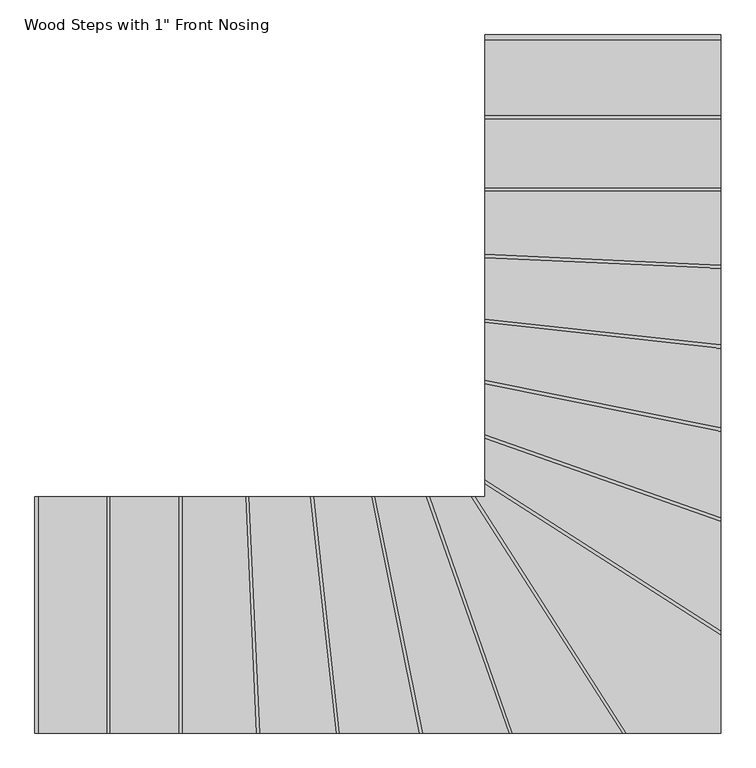
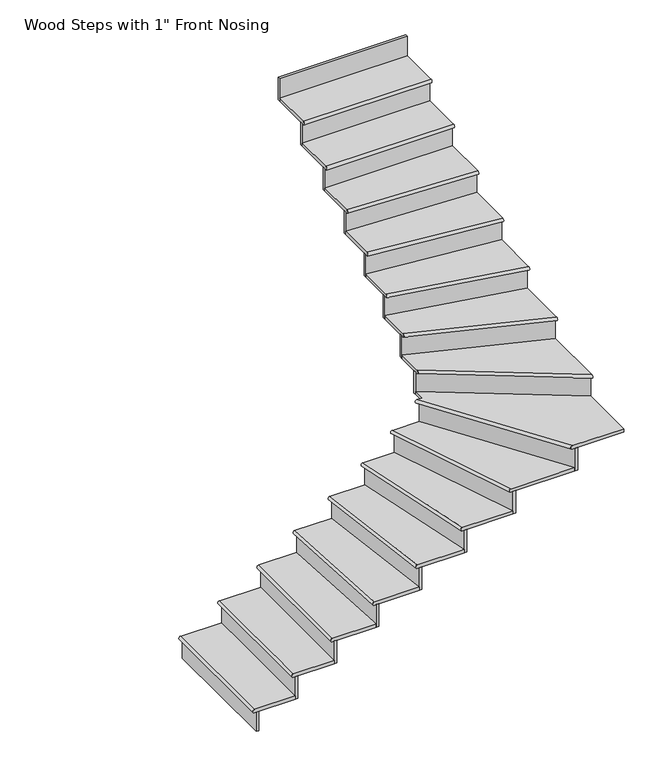
"""IFC4 building model written with IfcOpenShell, lengths in millimetres: stair flight geometry."""

from ifc_helpers import new_model, si_unit, frame, origin, place, context, project, spatial, circle_curve, ellipse_curve, faceted_brep, source, transform, mapped, element, save
from ifc_brep_helpers import plane_surface, cylinder_surface, advanced_brep


def stair_flight_5aa84afe(model_context):
    return source(origin(), model_context, "Body", "SolidModel", [
        advanced_brep(
        [(6790.9616192, -13389.0529211, 146.05), (6790.9616192, -13389.0529211, 171.45), (6790.9616192, -12474.6529211, 171.45), (6790.9616192, -12474.6529211, 146.05), (7083.0616192, -12474.6529211, 171.45), (7083.0616192, -13389.0529211, 171.45), (7083.0616192, -12474.6529211, 146.05), (7083.0616192, -13389.0529211, 146.05)],
        [
            (0, 1, circle_curve(frame((6790.9616192, -13389.0529211, 158.75), z_axis=(0.0, 1.0, 0.0), x_axis=(1.0, 0.0, 0.0)), 12.7)),
            (1, 2),
            (2, 3, circle_curve(frame((6790.9616192, -12474.6529211, 158.75), z_axis=(0.0, -1.0, 0.0), x_axis=(1.0, 0.0, 0.0)), 12.7)),
            (3, 0),
            (4, 2),
            (1, 5),
            (5, 4),
            (3, 6),
            (6, 7),
            (7, 0),
            (4, 6),
            (7, 5),
        ],
        [
            cylinder_surface(frame((6790.9616192, -13389.0529211, 158.75), z_axis=(0.0, -1.0, 0.0), x_axis=(1.0, 0.0, 0.0)), 12.7),
            plane_surface(frame((8977.5986087, -12474.6529211, 171.45), z_axis=(0.0, 0.0, 1.0), x_axis=(-1.0, 0.0, 0.0))),
            plane_surface(frame((8977.5986087, -12474.6529211, 146.05), z_axis=(0.0, 0.0, -1.0), x_axis=(1.0, 0.0, 0.0))),
            plane_surface(frame((7083.0616192, -12474.6529211, 171.45), z_axis=(0.0, 1.0, 0.0), x_axis=(0.0, 0.0, -1.0))),
            plane_surface(frame((6790.9616192, -13389.0529211, 171.45), z_axis=(0.0, -1.0, 0.0), x_axis=(0.0, 0.0, -1.0))),
            plane_surface(frame((7083.0616192, -13389.0529211, 171.45), z_axis=(1.0, 0.0, 0.0), x_axis=(0.0, 0.0, -1.0))),
        ],
        [
            (0, [[1, 2, 3, 4]]),
            (1, [[5, -2, 6, 7]]),
            (2, [[8, 9, 10, -4]]),
            (3, [[-5, 11, -8, -3]]),
            (4, [[-6, -1, -10, 12]]),
            (5, [[-7, -12, -9, -11]]),
        ],
    ),
        faceted_brep([(6803.6616192, -13389.0529211, 146.05), (6803.6616192, -13389.0529211, 0.0), (6822.7116192, -13389.0529211, 0.0), (6822.7116192, -13389.0529211, 146.05), (6803.6616192, -12474.6529211, 146.05), (6822.7116192, -12474.6529211, 146.05), (6822.7116192, -12474.6529211, 0.0), (6803.6616192, -12474.6529211, 0.0)], [[[0, 1, 2, 3]], [[4, 5, 6, 7]], [[1, 0, 4, 7]], [[2, 1, 7, 6]], [[3, 2, 6, 5]], [[0, 3, 5, 4]]]),
        faceted_brep([(7083.0616192, -13389.0529211, 317.5), (7083.0616192, -13389.0529211, 146.05), (7102.1116192, -13389.0529211, 146.05), (7102.1116192, -13389.0529211, 317.5), (7083.0616192, -12474.6529211, 317.5), (7102.1116192, -12474.6529211, 317.5), (7102.1116192, -12474.6529211, 146.05), (7083.0616192, -12474.6529211, 146.05)], [[[0, 1, 2, 3]], [[4, 5, 6, 7]], [[1, 0, 4, 7]], [[2, 1, 7, 6]], [[3, 2, 6, 5]], [[0, 3, 5, 4]]]),
        advanced_brep(
        [(7362.4616192, -12474.6529211, 342.9), (7070.3616192, -12474.6529211, 342.9), (7070.3616192, -13389.0529211, 342.9), (7362.4616192, -13389.0529211, 342.9), (7070.3616192, -12474.6529211, 317.5), (7362.4616192, -12474.6529211, 317.5), (7362.4616192, -13389.0529211, 317.5), (7070.3616192, -13389.0529211, 317.5)],
        [
            (0, 1),
            (1, 2),
            (2, 3),
            (3, 0),
            (4, 5),
            (5, 6),
            (6, 7),
            (7, 4),
            (0, 5),
            (4, 1, circle_curve(frame((7070.3616192, -12474.6529211, 330.2), z_axis=(0.0, 1.0, 0.0), x_axis=(1.0, 0.0, 0.0)), 12.7)),
            (2, 7, circle_curve(frame((7070.3616192, -13389.0529211, 330.2), z_axis=(0.0, -1.0, 0.0), x_axis=(1.0, 0.0, 0.0)), 12.7)),
            (6, 3),
        ],
        [
            plane_surface(frame((8977.5986087, -12474.6529211, 342.9), z_axis=(0.0, 0.0, 1.0), x_axis=(-1.0, 0.0, 0.0))),
            plane_surface(frame((8977.5986087, -12474.6529211, 317.5), z_axis=(0.0, 0.0, -1.0), x_axis=(1.0, 0.0, 0.0))),
            plane_surface(frame((7362.4616192, -12474.6529211, 342.9), z_axis=(0.0, 1.0, 0.0), x_axis=(0.0, 0.0, -1.0))),
            plane_surface(frame((7070.3616192, -13389.0529211, 342.9), z_axis=(0.0, -1.0, 0.0), x_axis=(0.0, 0.0, -1.0))),
            plane_surface(frame((7362.4616192, -13389.0529211, 342.9), z_axis=(1.0, 0.0, 0.0), x_axis=(0.0, 0.0, -1.0))),
            cylinder_surface(frame((7070.3616192, -13389.0529211, 330.2), z_axis=(0.0, -1.0, 0.0), x_axis=(1.0, 0.0, 0.0)), 12.7),
        ],
        [
            (0, [[1, 2, 3, 4]]),
            (1, [[5, 6, 7, 8]]),
            (2, [[-1, 9, -5, 10]]),
            (3, [[-3, 11, -7, 12]]),
            (4, [[-4, -12, -6, -9]]),
            (5, [[-11, -2, -10, -8]]),
        ],
    ),
        faceted_brep([(7362.4616192, -13389.0529211, 488.95), (7362.4616192, -13389.0529211, 317.5), (7381.5116192, -13389.0529211, 317.5), (7381.5116192, -13389.0529211, 488.95), (7362.4616192, -12474.6529211, 488.95), (7381.5116192, -12474.6529211, 488.95), (7381.5116192, -12474.6529211, 317.5), (7362.4616192, -12474.6529211, 317.5)], [[[0, 1, 2, 3]], [[4, 5, 6, 7]], [[1, 0, 4, 7]], [[2, 1, 7, 6]], [[3, 2, 6, 5]], [[0, 3, 5, 4]]]),
        advanced_brep(
        [(7620.8913889, -12474.6529211, 514.35), (7349.7616192, -12474.6529211, 514.35), (7349.7616192, -13389.0529211, 514.35), (7662.8853931, -13389.0529211, 514.35), (7349.7616192, -12474.6529211, 488.95), (7620.8913889, -12474.6529211, 488.95), (7662.8853931, -13389.0529211, 488.95), (7349.7616192, -13389.0529211, 488.95)],
        [
            (0, 1),
            (1, 2),
            (2, 3),
            (3, 0),
            (4, 5),
            (5, 6),
            (6, 7),
            (7, 4),
            (0, 5),
            (4, 1, circle_curve(frame((7349.7616192, -12474.6529211, 501.65), z_axis=(0.0, 1.0, 0.0), x_axis=(1.0, 0.0, 0.0)), 12.7)),
            (2, 7, circle_curve(frame((7349.7616192, -13389.0529211, 501.65), z_axis=(0.0, -1.0, 0.0), x_axis=(1.0, 0.0, 0.0)), 12.7)),
            (6, 3),
        ],
        [
            plane_surface(frame((8977.5986087, -12474.6529211, 514.35), z_axis=(0.0, 0.0, 1.0), x_axis=(-1.0, 0.0, 0.0))),
            plane_surface(frame((8977.5986087, -12474.6529211, 488.95), z_axis=(0.0, 0.0, -1.0), x_axis=(1.0, 0.0, 0.0))),
            plane_surface(frame((7620.8913889, -12474.6529211, 514.35), z_axis=(0.0, 1.0, 0.0), x_axis=(0.0, 0.0, -1.0))),
            plane_surface(frame((7349.7616192, -13389.0529211, 514.35), z_axis=(0.0, -1.0, 0.0), x_axis=(0.0, 0.0, -1.0))),
            plane_surface(frame((7662.8853931, -13389.0529211, 514.35), z_axis=(0.998947103163783, 0.04587684689128463, 0.0), x_axis=(0.0, 0.0, -1.0))),
            cylinder_surface(frame((7349.7616192, -13389.0529211, 501.65), z_axis=(0.0, -1.0, 0.0), x_axis=(1.0, 0.0, 0.0)), 12.7),
        ],
        [
            (0, [[1, 2, 3, 4]]),
            (1, [[5, 6, 7, 8]]),
            (2, [[-1, 9, -5, 10]]),
            (3, [[-3, 11, -7, 12]]),
            (4, [[-4, -12, -6, -9]]),
            (5, [[-11, -2, -10, -8]]),
        ],
    ),
        faceted_brep([(7662.8853931, -13389.0529211, 660.4), (7662.8853931, -13389.0529211, 488.95), (7681.9554719, -13389.0529211, 488.95), (7681.9554719, -13389.0529211, 660.4), (7620.8913889, -12474.6529211, 660.4), (7639.9614678, -12474.6529211, 660.4), (7639.9614678, -12474.6529211, 488.95), (7620.8913889, -12474.6529211, 488.95)], [[[0, 1, 2, 3]], [[4, 5, 6, 7]], [[1, 0, 4, 7]], [[2, 1, 7, 6]], [[3, 2, 6, 5]], [[0, 3, 5, 4]]]),
        advanced_brep(
        [(7871.5131081, -12474.6529211, 685.8), (7608.178003, -12474.6529211, 685.8), (7650.1720072, -13389.0529211, 685.8), (7971.3117943, -13389.0529211, 685.8), (7608.178003, -12474.6529211, 660.4), (7871.5131081, -12474.6529211, 660.4), (7971.3117943, -13389.0529211, 660.4), (7650.1720072, -13389.0529211, 660.4)],
        [
            (0, 1),
            (1, 2),
            (2, 3),
            (3, 0),
            (4, 5),
            (5, 6),
            (6, 7),
            (7, 4),
            (0, 5),
            (4, 1, ellipse_curve(frame((7608.178003, -12474.6529211, 673.1), z_axis=(0.0, 1.0, 0.0), x_axis=(1.0, 0.0, 0.0)), 12.7133859, 12.7)),
            (2, 7, ellipse_curve(frame((7650.1720072, -13389.0529211, 673.1), z_axis=(0.0, -1.0, 0.0), x_axis=(1.0, 0.0, 0.0)), 12.7133859, 12.7)),
            (6, 3),
        ],
        [
            plane_surface(frame((8977.5986087, -12474.6529211, 685.8), z_axis=(0.0, 0.0, 1.0), x_axis=(-1.0, 0.0, 0.0))),
            plane_surface(frame((8977.5986087, -12474.6529211, 660.4), z_axis=(0.0, 0.0, -1.0), x_axis=(1.0, 0.0, 0.0))),
            plane_surface(frame((7871.5131081, -12474.6529211, 685.8), z_axis=(0.0, 1.0, 0.0), x_axis=(0.0, 0.0, -1.0))),
            plane_surface(frame((7650.1720072, -13389.0529211, 685.8), z_axis=(0.0, -1.0, 0.0), x_axis=(0.0, 0.0, -1.0))),
            plane_surface(frame((7971.3117943, -13389.0529211, 685.8), z_axis=(0.9940967888076031, 0.10849688697106348, 0.0), x_axis=(0.0, 0.0, -1.0))),
            cylinder_surface(frame((7650.1720072, -13389.0529211, 673.1), z_axis=(0.04587684689128463, -0.998947103163783, 0.0), x_axis=(0.998947103163783, 0.04587684689128463, 0.0)), 12.7),
        ],
        [
            (0, [[1, 2, 3, 4]]),
            (1, [[5, 6, 7, 8]]),
            (2, [[-1, 9, -5, 10]]),
            (3, [[-3, 11, -7, 12]]),
            (4, [[-4, -12, -6, -9]]),
            (5, [[-11, -2, -10, -8]]),
        ],
    ),
        faceted_brep([(7971.3117943, -13389.0529211, 831.85), (7971.3117943, -13389.0529211, 660.4), (7990.4749182, -13389.0529211, 660.4), (7990.4749182, -13389.0529211, 831.85), (7871.5131081, -12474.6529211, 831.85), (7890.6762321, -12474.6529211, 831.85), (7890.6762321, -12474.6529211, 660.4), (7871.5131081, -12474.6529211, 660.4)], [[[0, 1, 2, 3]], [[4, 5, 6, 7]], [[1, 0, 4, 7]], [[2, 1, 7, 6]], [[3, 2, 6, 5]], [[0, 3, 5, 4]]]),
        advanced_brep(
        [(8108.9661368, -12474.6529211, 857.25), (7858.7376921, -12474.6529211, 857.25), (7958.5363783, -13389.0529211, 857.25), (8293.3799184, -13389.0529211, 857.25), (7858.7376921, -12474.6529211, 831.85), (8108.9661368, -12474.6529211, 831.85), (8293.3799184, -13389.0529211, 831.85), (7958.5363783, -13389.0529211, 831.85)],
        [
            (0, 1),
            (1, 2),
            (2, 3),
            (3, 0),
            (4, 5),
            (5, 6),
            (6, 7),
            (7, 4),
            (0, 5),
            (4, 1, ellipse_curve(frame((7858.7376921, -12474.6529211, 844.55), z_axis=(0.0, 1.0, 0.0), x_axis=(1.0, 0.0, 0.0)), 12.775416, 12.7)),
            (2, 7, ellipse_curve(frame((7958.5363783, -13389.0529211, 844.55), z_axis=(0.0, -1.0, 0.0), x_axis=(1.0, 0.0, 0.0)), 12.775416, 12.7)),
            (6, 3),
        ],
        [
            plane_surface(frame((8977.5986087, -12474.6529211, 857.25), z_axis=(0.0, 0.0, 1.0), x_axis=(-1.0, 0.0, 0.0))),
            plane_surface(frame((8977.5986087, -12474.6529211, 831.85), z_axis=(0.0, 0.0, -1.0), x_axis=(1.0, 0.0, 0.0))),
            plane_surface(frame((8108.9661368, -12474.6529211, 857.25), z_axis=(0.0, 1.0, 0.0), x_axis=(0.0, 0.0, -1.0))),
            plane_surface(frame((7958.5363783, -13389.0529211, 857.25), z_axis=(0.0, -1.0, 0.0), x_axis=(0.0, 0.0, -1.0))),
            plane_surface(frame((8293.3799184, -13389.0529211, 857.25), z_axis=(0.9802631976454906, 0.19769689765354914, 0.0), x_axis=(0.0, 0.0, -1.0))),
            cylinder_surface(frame((7958.5363783, -13389.0529211, 844.55), z_axis=(0.10849688697106348, -0.9940967888076031, 0.0), x_axis=(0.9940967888076031, 0.10849688697106348, 0.0)), 12.7),
        ],
        [
            (0, [[1, 2, 3, 4]]),
            (1, [[5, 6, 7, 8]]),
            (2, [[-1, 9, -5, 10]]),
            (3, [[-3, 11, -7, 12]]),
            (4, [[-4, -12, -6, -9]]),
            (5, [[-11, -2, -10, -8]]),
        ],
    ),
        faceted_brep([(8293.3799184, -13389.0529211, 1003.3), (8293.3799184, -13389.0529211, 831.85), (8312.8134746, -13389.0529211, 831.85), (8312.8134746, -13389.0529211, 1003.3), (8108.9661368, -12474.6529211, 1003.3), (8128.3996931, -12474.6529211, 1003.3), (8128.3996931, -12474.6529211, 831.85), (8108.9661368, -12474.6529211, 831.85)], [[[0, 1, 2, 3]], [[4, 5, 6, 7]], [[1, 0, 4, 7]], [[2, 1, 7, 6]], [[3, 2, 6, 5]], [[0, 3, 5, 4]]]),
        advanced_brep(
        [(8321.51155, -12474.6529211, 1028.7), (8096.0104326, -12474.6529211, 1028.7), (8280.4242142, -13389.0529211, 1028.7), (8641.6348525, -13389.0529211, 1028.7), (8096.0104326, -12474.6529211, 1003.3), (8321.51155, -12474.6529211, 1003.3), (8641.6348525, -13389.0529211, 1003.3), (8280.4242142, -13389.0529211, 1003.3)],
        [
            (0, 1),
            (1, 2),
            (2, 3),
            (3, 0),
            (4, 5),
            (5, 6),
            (6, 7),
            (7, 4),
            (0, 5),
            (4, 1, ellipse_curve(frame((8096.0104326, -12474.6529211, 1016.0), z_axis=(0.0, 1.0, 0.0), x_axis=(1.0, 0.0, 0.0)), 12.9557042, 12.7)),
            (2, 7, ellipse_curve(frame((8280.4242142, -13389.0529211, 1016.0), z_axis=(0.0, -1.0, 0.0), x_axis=(1.0, 0.0, 0.0)), 12.9557042, 12.7)),
            (6, 3),
        ],
        [
            plane_surface(frame((8977.5986087, -12474.6529211, 1028.7), z_axis=(0.0, 0.0, 1.0), x_axis=(-1.0, 0.0, 0.0))),
            plane_surface(frame((8977.5986087, -12474.6529211, 1003.3), z_axis=(0.0, 0.0, -1.0), x_axis=(1.0, 0.0, 0.0))),
            plane_surface(frame((8321.51155, -12474.6529211, 1028.7), z_axis=(0.0, 1.0, 0.0), x_axis=(0.0, 0.0, -1.0))),
            plane_surface(frame((8280.4242142, -13389.0529211, 1028.7), z_axis=(0.0, -1.0, 0.0), x_axis=(0.0, 0.0, -1.0))),
            plane_surface(frame((8641.6348525, -13389.0529211, 1028.7), z_axis=(0.9438315431717413, 0.33042702388583395, 0.0), x_axis=(0.0, 0.0, -1.0))),
            cylinder_surface(frame((8280.4242142, -13389.0529211, 1016.0), z_axis=(0.19769689765354914, -0.9802631976454906, 0.0), x_axis=(0.9802631976454906, 0.19769689765354914, 0.0)), 12.7),
        ],
        [
            (0, [[1, 2, 3, 4]]),
            (1, [[5, 6, 7, 8]]),
            (2, [[-1, 9, -5, 10]]),
            (3, [[-3, 11, -7, 12]]),
            (4, [[-4, -12, -6, -9]]),
            (5, [[-11, -2, -10, -8]]),
        ],
    ),
        faceted_brep([(8641.6348525, -13389.0529211, 1174.75), (8641.6348525, -13389.0529211, 1003.3), (8661.8185391, -13389.0529211, 1003.3), (8661.8185391, -13389.0529211, 1174.75), (8321.51155, -12474.6529211, 1174.75), (8341.6952365, -12474.6529211, 1174.75), (8341.6952365, -12474.6529211, 1003.3), (8321.51155, -12474.6529211, 1003.3)], [[[0, 1, 2, 3]], [[4, 5, 6, 7]], [[1, 0, 4, 7]], [[2, 1, 7, 6]], [[3, 2, 6, 5]], [[0, 3, 5, 4]]]),
        advanced_brep(
        [(8499.6342421, -12474.6529211, 1200.15), (8308.055759, -12474.6529211, 1200.15), (8628.1790615, -13389.0529211, 1200.15), (9084.2336776, -13389.0529211, 1200.15), (8308.055759, -12474.6529211, 1174.75), (8499.6342421, -12474.6529211, 1174.75), (9084.2336776, -13389.0529211, 1174.75), (8628.1790615, -13389.0529211, 1174.75)],
        [
            (0, 1),
            (1, 2),
            (2, 3),
            (3, 0),
            (4, 5),
            (5, 6),
            (6, 7),
            (7, 4),
            (0, 5),
            (4, 1, ellipse_curve(frame((8308.055759, -12474.6529211, 1187.45), z_axis=(0.0, 1.0, 0.0), x_axis=(0.9999999999999999, 0.0, 0.0)), 13.455791, 12.7)),
            (2, 7, ellipse_curve(frame((8628.1790615, -13389.0529211, 1187.45), z_axis=(0.0, -1.0, 0.0), x_axis=(0.9999999999999999, 0.0, 0.0)), 13.455791, 12.7)),
            (6, 3),
        ],
        [
            plane_surface(frame((8977.5986087, -12474.6529211, 1200.15), z_axis=(0.0, 0.0, 1.0), x_axis=(-1.0, 0.0, 0.0))),
            plane_surface(frame((8977.5986087, -12474.6529211, 1174.75), z_axis=(0.0, 0.0, -1.0), x_axis=(1.0, 0.0, 0.0))),
            plane_surface(frame((8499.6342421, -12474.6529211, 1200.15), z_axis=(0.0, 1.0, 0.0), x_axis=(0.0, 0.0, -1.0))),
            plane_surface(frame((8628.1790615, -13389.0529211, 1200.15), z_axis=(0.0, -1.0, 0.0), x_axis=(0.0, 0.0, -1.0))),
            plane_surface(frame((9084.2336776, -13389.0529211, 1200.15), z_axis=(0.8425292399238443, 0.5386506102041927, 0.0), x_axis=(0.0, 0.0, -1.0))),
            cylinder_surface(frame((8628.1790615, -13389.0529211, 1187.45), z_axis=(0.33042702388583395, -0.9438315431717413, 0.0), x_axis=(0.9438315431717413, 0.33042702388583395, 0.0)), 12.7),
        ],
        [
            (0, [[1, 2, 3, 4]]),
            (1, [[5, 6, 7, 8]]),
            (2, [[-1, 9, -5, 10]]),
            (3, [[-3, 11, -7, 12]]),
            (4, [[-4, -12, -6, -9]]),
            (5, [[-11, -2, -10, -8]]),
        ],
    ),
        faceted_brep([(9084.2336776, -13389.0529211, 1346.2), (9084.2336776, -13389.0529211, 1174.75), (9106.8441688, -13389.0529211, 1174.75), (9106.8441688, -13389.0529211, 1346.2), (8499.6342421, -12474.6529211, 1346.2), (8522.2447334, -12474.6529211, 1346.2), (8522.2447334, -12474.6529211, 1174.75), (8499.6342421, -12474.6529211, 1174.75)], [[[0, 1, 2, 3]], [[4, 5, 6, 7]], [[1, 0, 4, 7]], [[2, 1, 7, 6]], [[3, 2, 6, 5]], [[0, 3, 5, 4]]]),
        advanced_brep(
        [(8520.3986087, -12393.5939112, 1371.6), (8520.3986087, -12474.6529211, 1371.6), (8484.5605813, -12474.6529211, 1371.6), (9069.1600167, -13389.0529211, 1371.6), (9434.7986087, -13389.0529211, 1371.6), (9434.7986087, -12978.1933466, 1371.6), (8520.3986087, -12474.6529211, 1346.2), (8520.3986087, -12393.5939112, 1346.2), (9434.7986087, -12978.1933466, 1346.2), (9434.7986087, -13389.0529211, 1346.2), (9069.1600167, -13389.0529211, 1346.2), (8484.5605813, -12474.6529211, 1346.2)],
        [
            (0, 1),
            (1, 2),
            (2, 3),
            (3, 4),
            (4, 5),
            (5, 0),
            (6, 7),
            (7, 8),
            (8, 9),
            (9, 10),
            (10, 11),
            (11, 6),
            (0, 7),
            (6, 1),
            (11, 2, ellipse_curve(frame((8484.5605813, -12474.6529211, 1358.9), z_axis=(0.0, 1.0, 0.0), x_axis=(1.0, 0.0, 0.0)), 15.0736608, 12.7)),
            (3, 10, ellipse_curve(frame((9069.1600167, -13389.0529211, 1358.9), z_axis=(0.0, -1.0, 0.0), x_axis=(1.0, 0.0, 0.0)), 15.0736608, 12.7)),
            (9, 4),
            (8, 5),
        ],
        [
            plane_surface(frame((8520.3986087, -10732.5159316, 1371.6), z_axis=(0.0, 0.0, 1.0), x_axis=(0.0, -1.0, 0.0))),
            plane_surface(frame((8520.3986087, -10732.5159316, 1346.2), z_axis=(0.0, 0.0, -1.0), x_axis=(0.0, 1.0, 0.0))),
            plane_surface(frame((8520.3986087, -12393.5939112, 1371.6), z_axis=(-1.0, 0.0, 0.0), x_axis=(0.0, 0.0, -1.0))),
            plane_surface(frame((8520.3986087, -12474.6529211, 1371.6), z_axis=(0.0, 1.0, 0.0), x_axis=(0.0, 0.0, -1.0))),
            plane_surface(frame((9069.1600167, -13389.0529211, 1371.6), z_axis=(0.0, -1.0, 0.0), x_axis=(0.0, 0.0, -1.0))),
            plane_surface(frame((9434.7986087, -13389.0529211, 1371.6), z_axis=(1.0, 0.0, 0.0), x_axis=(0.0, 0.0, -1.0))),
            plane_surface(frame((9434.7986087, -12978.1933466, 1371.6), z_axis=(0.538650610204191, 0.8425292399238455, 0.0), x_axis=(0.0, 0.0, -1.0))),
            cylinder_surface(frame((9069.1600167, -13389.0529211, 1358.9), z_axis=(0.5386506102041927, -0.8425292399238443, 0.0), x_axis=(0.8425292399238443, 0.5386506102041927, 0.0)), 12.7),
        ],
        [
            (0, [[1, 2, 3, 4, 5, 6]]),
            (1, [[7, 8, 9, 10, 11, 12]]),
            (2, [[-1, 13, -7, 14]]),
            (3, [[-2, -14, -12, 15]]),
            (4, [[-4, 16, -10, 17]]),
            (5, [[-5, -17, -9, 18]]),
            (6, [[-6, -18, -8, -13]]),
            (7, [[-16, -3, -15, -11]]),
        ],
    ),
        faceted_brep([(9434.7986087, -12978.1933466, 1517.65), (9434.7986087, -12978.1933466, 1346.2), (9434.7986087, -12955.5828554, 1346.2), (9434.7986087, -12955.5828554, 1517.65), (8520.3986087, -12393.5939112, 1517.65), (8520.3986087, -12370.98342, 1517.65), (8520.3986087, -12370.98342, 1346.2), (8520.3986087, -12393.5939112, 1346.2)], [[[0, 1, 2, 3]], [[4, 5, 6, 7]], [[1, 0, 4, 7]], [[2, 1, 7, 6]], [[3, 2, 6, 5]], [[0, 3, 5, 4]]]),
        advanced_brep(
        [(8520.3986087, -12221.9426983, 1543.05), (8520.3986087, -12408.6675721, 1543.05), (9434.7986087, -12993.2670075, 1543.05), (9434.7986087, -12542.0660009, 1543.05), (8520.3986087, -12408.6675721, 1517.65), (8520.3986087, -12221.9426983, 1517.65), (9434.7986087, -12542.0660009, 1517.65), (9434.7986087, -12993.2670075, 1517.65)],
        [
            (0, 1),
            (1, 2),
            (2, 3),
            (3, 0),
            (4, 5),
            (5, 6),
            (6, 7),
            (7, 4),
            (0, 5),
            (4, 1, ellipse_curve(frame((8520.3986087, -12408.6675721, 1530.35), z_axis=(-1.0, 0.0, 0.0), x_axis=(0.0, -1.0, 0.0)), 15.0736608, 12.7)),
            (2, 7, ellipse_curve(frame((9434.7986087, -12993.2670075, 1530.35), z_axis=(1.0, 0.0, 0.0), x_axis=(0.0, -1.0, 0.0)), 15.0736608, 12.7)),
            (6, 3),
        ],
        [
            plane_surface(frame((8520.3986087, -10732.5159316, 1543.05), z_axis=(0.0, 0.0, 1.0), x_axis=(0.0, -1.0, 0.0))),
            plane_surface(frame((8520.3986087, -10732.5159316, 1517.65), z_axis=(0.0, 0.0, -1.0), x_axis=(0.0, 1.0, 0.0))),
            plane_surface(frame((8520.3986087, -12221.9426983, 1543.05), z_axis=(-1.0, 0.0, 0.0), x_axis=(0.0, 0.0, -1.0))),
            plane_surface(frame((9434.7986087, -12993.2670075, 1543.05), z_axis=(1.0, 0.0, 0.0), x_axis=(0.0, 0.0, -1.0))),
            plane_surface(frame((9434.7986087, -12542.0660009, 1543.05), z_axis=(0.33042702388583306, 0.9438315431717417, 0.0), x_axis=(0.0, 0.0, -1.0))),
            cylinder_surface(frame((9434.7986087, -12993.2670075, 1530.35), z_axis=(0.8425292399238455, -0.538650610204191, 0.0), x_axis=(0.538650610204191, 0.8425292399238455, 0.0)), 12.7),
        ],
        [
            (0, [[1, 2, 3, 4]]),
            (1, [[5, 6, 7, 8]]),
            (2, [[-1, 9, -5, 10]]),
            (3, [[-3, 11, -7, 12]]),
            (4, [[-4, -12, -6, -9]]),
            (5, [[-11, -2, -10, -8]]),
        ],
    ),
        faceted_brep([(9434.7986087, -12542.0660009, 1689.1), (9434.7986087, -12542.0660009, 1517.65), (9434.7986087, -12521.8823144, 1517.65), (9434.7986087, -12521.8823144, 1689.1), (8520.3986087, -12221.9426983, 1689.1), (8520.3986087, -12201.7590118, 1689.1), (8520.3986087, -12201.7590118, 1517.65), (8520.3986087, -12221.9426983, 1517.65)], [[[0, 1, 2, 3]], [[4, 5, 6, 7]], [[1, 0, 4, 7]], [[2, 1, 7, 6]], [[3, 2, 6, 5]], [[0, 3, 5, 4]]]),
        advanced_brep(
        [(8520.3986087, -12011.3976325, 1714.5), (8520.3986087, -12235.3984894, 1714.5), (9434.7986087, -12555.5217919, 1714.5), (9434.7986087, -12195.8114141, 1714.5), (8520.3986087, -12235.3984894, 1689.1), (8520.3986087, -12011.3976325, 1689.1), (9434.7986087, -12195.8114141, 1689.1), (9434.7986087, -12555.5217919, 1689.1)],
        [
            (0, 1),
            (1, 2),
            (2, 3),
            (3, 0),
            (4, 5),
            (5, 6),
            (6, 7),
            (7, 4),
            (0, 5),
            (4, 1, ellipse_curve(frame((8520.3986087, -12235.3984894, 1701.8), z_axis=(-1.0, 0.0, 0.0), x_axis=(0.0, -1.0, 0.0)), 13.455791, 12.7)),
            (2, 7, ellipse_curve(frame((9434.7986087, -12555.5217919, 1701.8), z_axis=(1.0, 0.0, 0.0), x_axis=(0.0, -1.0, 0.0)), 13.455791, 12.7)),
            (6, 3),
        ],
        [
            plane_surface(frame((8520.3986087, -10732.5159316, 1714.5), z_axis=(0.0, 0.0, 1.0), x_axis=(0.0, -1.0, 0.0))),
            plane_surface(frame((8520.3986087, -10732.5159316, 1689.1), z_axis=(0.0, 0.0, -1.0), x_axis=(0.0, 1.0, 0.0))),
            plane_surface(frame((8520.3986087, -12011.3976325, 1714.5), z_axis=(-1.0, 0.0, 0.0), x_axis=(0.0, 0.0, -1.0))),
            plane_surface(frame((9434.7986087, -12555.5217919, 1714.5), z_axis=(1.0, 0.0, 0.0), x_axis=(0.0, 0.0, -1.0))),
            plane_surface(frame((9434.7986087, -12195.8114141, 1714.5), z_axis=(0.1976968976535497, 0.9802631976454905, 0.0), x_axis=(0.0, 0.0, -1.0))),
            cylinder_surface(frame((9434.7986087, -12555.5217919, 1701.8), z_axis=(0.9438315431717417, -0.33042702388583306, 0.0), x_axis=(0.33042702388583306, 0.9438315431717417, 0.0)), 12.7),
        ],
        [
            (0, [[1, 2, 3, 4]]),
            (1, [[5, 6, 7, 8]]),
            (2, [[-1, 9, -5, 10]]),
            (3, [[-3, 11, -7, 12]]),
            (4, [[-4, -12, -6, -9]]),
            (5, [[-11, -2, -10, -8]]),
        ],
    ),
        faceted_brep([(9434.7986087, -12195.8114141, 1860.55), (9434.7986087, -12195.8114141, 1689.1), (9434.7986087, -12176.3778578, 1689.1), (9434.7986087, -12176.3778578, 1860.55), (8520.3986087, -12011.3976325, 1860.55), (8520.3986087, -11991.9640763, 1860.55), (8520.3986087, -11991.9640763, 1689.1), (8520.3986087, -12011.3976325, 1689.1)], [[[0, 1, 2, 3]], [[4, 5, 6, 7]], [[1, 0, 4, 7]], [[2, 1, 7, 6]], [[3, 2, 6, 5]], [[0, 3, 5, 4]]]),
        advanced_brep(
        [(8520.3986087, -11774.6657566, 1885.95), (8520.3986087, -12024.3533367, 1885.95), (9434.7986087, -12208.7671183, 1885.95), (9434.7986087, -11874.4644428, 1885.95), (8520.3986087, -12024.3533367, 1860.55), (8520.3986087, -11774.6657566, 1860.55), (9434.7986087, -11874.4644428, 1860.55), (9434.7986087, -12208.7671183, 1860.55)],
        [
            (0, 1),
            (1, 2),
            (2, 3),
            (3, 0),
            (4, 5),
            (5, 6),
            (6, 7),
            (7, 4),
            (0, 5),
            (4, 1, ellipse_curve(frame((8520.3986087, -12024.3533367, 1873.25), z_axis=(-1.0, 0.0, 0.0), x_axis=(0.0, -1.0, 0.0)), 12.9557042, 12.7)),
            (2, 7, ellipse_curve(frame((9434.7986087, -12208.7671183, 1873.25), z_axis=(1.0, 0.0, 0.0), x_axis=(0.0, -1.0, 0.0)), 12.9557042, 12.7)),
            (6, 3),
        ],
        [
            plane_surface(frame((8520.3986087, -10732.5159316, 1885.95), z_axis=(0.0, 0.0, 1.0), x_axis=(0.0, -1.0, 0.0))),
            plane_surface(frame((8520.3986087, -10732.5159316, 1860.55), z_axis=(0.0, 0.0, -1.0), x_axis=(0.0, 1.0, 0.0))),
            plane_surface(frame((8520.3986087, -11774.6657566, 1885.95), z_axis=(-1.0, 0.0, 0.0), x_axis=(0.0, 0.0, -1.0))),
            plane_surface(frame((9434.7986087, -12208.7671183, 1885.95), z_axis=(1.0, 0.0, 0.0), x_axis=(0.0, 0.0, -1.0))),
            plane_surface(frame((9434.7986087, -11874.4644428, 1885.95), z_axis=(0.10849688697106538, 0.994096788807603, 0.0), x_axis=(0.0, 0.0, -1.0))),
            cylinder_surface(frame((9434.7986087, -12208.7671183, 1873.25), z_axis=(0.9802631976454905, -0.1976968976535497, 0.0), x_axis=(0.1976968976535497, 0.9802631976454905, 0.0)), 12.7),
        ],
        [
            (0, [[1, 2, 3, 4]]),
            (1, [[5, 6, 7, 8]]),
            (2, [[-1, 9, -5, 10]]),
            (3, [[-3, 11, -7, 12]]),
            (4, [[-4, -12, -6, -9]]),
            (5, [[-11, -2, -10, -8]]),
        ],
    ),
        faceted_brep([(9434.7986087, -11874.4644428, 2032.0), (9434.7986087, -11874.4644428, 1860.55), (9434.7986087, -11855.3013188, 1860.55), (9434.7986087, -11855.3013188, 2032.0), (8520.3986087, -11774.6657566, 2032.0), (8520.3986087, -11755.5026326, 2032.0), (8520.3986087, -11755.5026326, 1860.55), (8520.3986087, -11774.6657566, 1860.55)], [[[0, 1, 2, 3]], [[4, 5, 6, 7]], [[1, 0, 4, 7]], [[2, 1, 7, 6]], [[3, 2, 6, 5]], [[0, 3, 5, 4]]]),
        advanced_brep(
        [(8520.3986087, -11524.2921578, 2057.4), (8520.3986087, -11787.4411726, 2057.4), (9434.7986087, -11887.2398588, 2057.4), (9434.7986087, -11566.286162, 2057.4), (8520.3986087, -11787.4411726, 2032.0), (8520.3986087, -11524.2921578, 2032.0), (9434.7986087, -11566.286162, 2032.0), (9434.7986087, -11887.2398588, 2032.0)],
        [
            (0, 1),
            (1, 2),
            (2, 3),
            (3, 0),
            (4, 5),
            (5, 6),
            (6, 7),
            (7, 4),
            (0, 5),
            (4, 1, ellipse_curve(frame((8520.3986087, -11787.4411726, 2044.7), z_axis=(-1.0, 0.0, 0.0), x_axis=(0.0, -0.9999999999999999, 0.0)), 12.775416, 12.7)),
            (2, 7, ellipse_curve(frame((9434.7986087, -11887.2398588, 2044.7), z_axis=(1.0, 0.0, 0.0), x_axis=(0.0, -0.9999999999999999, 0.0)), 12.775416, 12.7)),
            (6, 3),
        ],
        [
            plane_surface(frame((8520.3986087, -10732.5159316, 2057.4), z_axis=(0.0, 0.0, 1.0), x_axis=(0.0, -1.0, 0.0))),
            plane_surface(frame((8520.3986087, -10732.5159316, 2032.0), z_axis=(0.0, 0.0, -1.0), x_axis=(0.0, 1.0, 0.0))),
            plane_surface(frame((8520.3986087, -11524.2921578, 2057.4), z_axis=(-1.0, 0.0, 0.0), x_axis=(0.0, 0.0, -1.0))),
            plane_surface(frame((9434.7986087, -11887.2398588, 2057.4), z_axis=(1.0, 0.0, 0.0), x_axis=(0.0, 0.0, -1.0))),
            plane_surface(frame((9434.7986087, -11566.286162, 2057.4), z_axis=(0.045876846891286835, 0.9989471031637829, 0.0), x_axis=(0.0, 0.0, -1.0))),
            cylinder_surface(frame((9434.7986087, -11887.2398588, 2044.7), z_axis=(0.994096788807603, -0.10849688697106538, 0.0), x_axis=(0.10849688697106538, 0.994096788807603, 0.0)), 12.7),
        ],
        [
            (0, [[1, 2, 3, 4]]),
            (1, [[5, 6, 7, 8]]),
            (2, [[-1, 9, -5, 10]]),
            (3, [[-3, 11, -7, 12]]),
            (4, [[-4, -12, -6, -9]]),
            (5, [[-11, -2, -10, -8]]),
        ],
    ),
        faceted_brep([(9434.7986087, -11566.286162, 2203.45), (9434.7986087, -11566.286162, 2032.0), (9434.7986087, -11547.2160831, 2032.0), (9434.7986087, -11547.2160831, 2203.45), (8520.3986087, -11524.2921578, 2203.45), (8520.3986087, -11505.222079, 2203.45), (8520.3986087, -11505.222079, 2032.0), (8520.3986087, -11524.2921578, 2032.0)], [[[0, 1, 2, 3]], [[4, 5, 6, 7]], [[1, 0, 4, 7]], [[2, 1, 7, 6]], [[3, 2, 6, 5]], [[0, 3, 5, 4]]]),
        advanced_brep(
        [(8520.3986087, -11265.9159316, 2228.85), (8520.3986087, -11537.0055437, 2228.85), (9434.7986087, -11578.9995478, 2228.85), (9434.7986087, -11265.9159316, 2228.85), (8520.3986087, -11537.0055437, 2203.45), (8520.3986087, -11265.9159316, 2203.45), (9434.7986087, -11265.9159316, 2203.45), (9434.7986087, -11578.9995478, 2203.45)],
        [
            (0, 1),
            (1, 2),
            (2, 3),
            (3, 0),
            (4, 5),
            (5, 6),
            (6, 7),
            (7, 4),
            (0, 5),
            (4, 1, ellipse_curve(frame((8520.3986087, -11537.0055437, 2216.15), z_axis=(-1.0, 0.0, 0.0), x_axis=(0.0, -1.0, 0.0)), 12.7133859, 12.7)),
            (2, 7, ellipse_curve(frame((9434.7986087, -11578.9995478, 2216.15), z_axis=(1.0, 0.0, 0.0), x_axis=(0.0, -1.0, 0.0)), 12.7133859, 12.7)),
            (6, 3),
        ],
        [
            plane_surface(frame((8520.3986087, -10732.5159316, 2228.85), z_axis=(0.0, 0.0, 1.0), x_axis=(0.0, -1.0, 0.0))),
            plane_surface(frame((8520.3986087, -10732.5159316, 2203.45), z_axis=(0.0, 0.0, -1.0), x_axis=(0.0, 1.0, 0.0))),
            plane_surface(frame((8520.3986087, -11265.9159316, 2228.85), z_axis=(-1.0, 0.0, 0.0), x_axis=(0.0, 0.0, -1.0))),
            plane_surface(frame((9434.7986087, -11578.9995478, 2228.85), z_axis=(1.0, 0.0, 0.0), x_axis=(0.0, 0.0, -1.0))),
            plane_surface(frame((9434.7986087, -11265.9159316, 2228.85), z_axis=(0.0, 1.0, 0.0), x_axis=(0.0, 0.0, -1.0))),
            cylinder_surface(frame((9434.7986087, -11578.9995478, 2216.15), z_axis=(0.9989471031637829, -0.045876846891286835, 0.0), x_axis=(0.045876846891286835, 0.9989471031637829, 0.0)), 12.7),
        ],
        [
            (0, [[1, 2, 3, 4]]),
            (1, [[5, 6, 7, 8]]),
            (2, [[-1, 9, -5, 10]]),
            (3, [[-3, 11, -7, 12]]),
            (4, [[-4, -12, -6, -9]]),
            (5, [[-11, -2, -10, -8]]),
        ],
    ),
        faceted_brep([(9434.7986087, -11265.9159316, 2374.9), (9434.7986087, -11265.9159316, 2203.45), (9434.7986087, -11246.8659316, 2203.45), (9434.7986087, -11246.8659316, 2374.9), (8520.3986087, -11265.9159316, 2374.9), (8520.3986087, -11246.8659316, 2374.9), (8520.3986087, -11246.8659316, 2203.45), (8520.3986087, -11265.9159316, 2203.45)], [[[0, 1, 2, 3]], [[4, 5, 6, 7]], [[1, 0, 4, 7]], [[2, 1, 7, 6]], [[3, 2, 6, 5]], [[0, 3, 5, 4]]]),
        advanced_brep(
        [(8520.3986087, -10986.5159316, 2400.3), (8520.3986087, -11278.6159316, 2400.3), (9434.7986087, -11278.6159316, 2400.3), (9434.7986087, -10986.5159316, 2400.3), (8520.3986087, -11278.6159316, 2374.9), (8520.3986087, -10986.5159316, 2374.9), (9434.7986087, -10986.5159316, 2374.9), (9434.7986087, -11278.6159316, 2374.9)],
        [
            (0, 1),
            (1, 2),
            (2, 3),
            (3, 0),
            (4, 5),
            (5, 6),
            (6, 7),
            (7, 4),
            (0, 5),
            (4, 1, circle_curve(frame((8520.3986087, -11278.6159316, 2387.6), z_axis=(-1.0, 0.0, 0.0), x_axis=(0.0, 1.0, 0.0)), 12.7)),
            (2, 7, circle_curve(frame((9434.7986087, -11278.6159316, 2387.6), z_axis=(1.0, 0.0, 0.0), x_axis=(0.0, 1.0, 0.0)), 12.7)),
            (6, 3),
        ],
        [
            plane_surface(frame((8520.3986087, -10732.5159316, 2400.3), z_axis=(0.0, 0.0, 1.0), x_axis=(0.0, -1.0, 0.0))),
            plane_surface(frame((8520.3986087, -10732.5159316, 2374.9), z_axis=(0.0, 0.0, -1.0), x_axis=(0.0, 1.0, 0.0))),
            plane_surface(frame((8520.3986087, -10986.5159316, 2400.3), z_axis=(-1.0, 0.0, 0.0), x_axis=(0.0, 0.0, -1.0))),
            plane_surface(frame((9434.7986087, -11278.6159316, 2400.3), z_axis=(1.0, 0.0, 0.0), x_axis=(0.0, 0.0, -1.0))),
            plane_surface(frame((9434.7986087, -10986.5159316, 2400.3), z_axis=(0.0, 1.0, 0.0), x_axis=(0.0, 0.0, -1.0))),
            cylinder_surface(frame((9434.7986087, -11278.6159316, 2387.6), z_axis=(1.0, 0.0, 0.0), x_axis=(0.0, 1.0, 0.0)), 12.7),
        ],
        [
            (0, [[1, 2, 3, 4]]),
            (1, [[5, 6, 7, 8]]),
            (2, [[-1, 9, -5, 10]]),
            (3, [[-3, 11, -7, 12]]),
            (4, [[-4, -12, -6, -9]]),
            (5, [[-11, -2, -10, -8]]),
        ],
    ),
        faceted_brep([(9434.7986087, -10986.5159316, 2546.35), (9434.7986087, -10986.5159316, 2374.9), (9434.7986087, -10967.4659316, 2374.9), (9434.7986087, -10967.4659316, 2546.35), (8520.3986087, -10986.5159316, 2546.35), (8520.3986087, -10967.4659316, 2546.35), (8520.3986087, -10967.4659316, 2374.9), (8520.3986087, -10986.5159316, 2374.9)], [[[0, 1, 2, 3]], [[4, 5, 6, 7]], [[1, 0, 4, 7]], [[2, 1, 7, 6]], [[3, 2, 6, 5]], [[0, 3, 5, 4]]]),
        faceted_brep([(9434.7986087, -10707.1159316, 2717.8), (9434.7986087, -10707.1159316, 2546.35), (9434.7986087, -10688.0659316, 2546.35), (9434.7986087, -10688.0659316, 2717.8), (8520.3986087, -10707.1159316, 2717.8), (8520.3986087, -10688.0659316, 2717.8), (8520.3986087, -10688.0659316, 2546.35), (8520.3986087, -10707.1159316, 2546.35)], [[[0, 1, 2, 3]], [[4, 5, 6, 7]], [[1, 0, 4, 7]], [[2, 1, 7, 6]], [[3, 2, 6, 5]], [[0, 3, 5, 4]]]),
        advanced_brep(
        [(8520.3986087, -10707.1159316, 2571.75), (8520.3986087, -10999.2159316, 2571.75), (9434.7986087, -10999.2159316, 2571.75), (9434.7986087, -10707.1159316, 2571.75), (8520.3986087, -10999.2159316, 2546.35), (8520.3986087, -10707.1159316, 2546.35), (9434.7986087, -10707.1159316, 2546.35), (9434.7986087, -10999.2159316, 2546.35)],
        [
            (0, 1),
            (1, 2),
            (2, 3),
            (3, 0),
            (4, 5),
            (5, 6),
            (6, 7),
            (7, 4),
            (0, 5),
            (4, 1, circle_curve(frame((8520.3986087, -10999.2159316, 2559.05), z_axis=(-1.0, 0.0, 0.0), x_axis=(0.0, 1.0, 0.0)), 12.7)),
            (2, 7, circle_curve(frame((9434.7986087, -10999.2159316, 2559.05), z_axis=(1.0, 0.0, 0.0), x_axis=(0.0, 1.0, 0.0)), 12.7)),
            (6, 3),
        ],
        [
            plane_surface(frame((8520.3986087, -10453.1159316, 2571.75), z_axis=(0.0, 0.0, 1.0), x_axis=(0.0, -1.0, 0.0))),
            plane_surface(frame((8520.3986087, -10453.1159316, 2546.35), z_axis=(0.0, 0.0, -1.0), x_axis=(0.0, 1.0, 0.0))),
            plane_surface(frame((8520.3986087, -10707.1159316, 2571.75), z_axis=(-1.0, 0.0, 0.0), x_axis=(0.0, 0.0, -1.0))),
            plane_surface(frame((9434.7986087, -10999.2159316, 2571.75), z_axis=(1.0, 0.0, 0.0), x_axis=(0.0, 0.0, -1.0))),
            plane_surface(frame((9434.7986087, -10707.1159316, 2571.75), z_axis=(0.0, 1.0, 0.0), x_axis=(0.0, 0.0, -1.0))),
            cylinder_surface(frame((9434.7986087, -10999.2159316, 2559.05), z_axis=(1.0, 0.0, 0.0), x_axis=(0.0, 1.0, 0.0)), 12.7),
        ],
        [
            (0, [[1, 2, 3, 4]]),
            (1, [[5, 6, 7, 8]]),
            (2, [[-1, 9, -5, 10]]),
            (3, [[-3, 11, -7, 12]]),
            (4, [[-4, -12, -6, -9]]),
            (5, [[-11, -2, -10, -8]]),
        ],
    ),
    ])


if __name__ == "__main__":
    model = new_model("IFC4")
    model_context = context("Model", 3, world=origin())
    ifc_project = project(units=[si_unit("LENGTHUNIT", "METRE", prefix="MILLI")], contexts=[model_context])
    site = spatial("IfcSite", under=ifc_project)
    building = spatial("IfcBuilding", under=site)
    placement = place(None, origin())
    stair_flight_shape = stair_flight_5aa84afe(model_context)
    element("IfcStairFlight", 1, ObjectType="Wood Steps with 1\" Front Nosing", at=placement, inside=building, context=model_context, shape_type="MappedRepresentation", body=[
        mapped(stair_flight_shape, transform((0.0, 0.0, 0.0), x_axis=(1.0, 0.0, 0.0), y_axis=(0.0, 1.0, 0.0), z_axis=(0.0, 0.0, 1.0))),
    ])
    save(model, "model.ifc")

# Revit data of these elements
# Element 1 (IfcStairFlight, "Wood Steps with 1\" Front Nosing")
#   Materials on its faces: "Paints and Coatings", "Cherry"
# Materials
#   "Paints and Coatings": class "Paint", colour RGB 244 244 244, transparency 0, Description = "Interior finish", Cost = 0
#   "Cherry": class "Wood", colour RGB 233 182 144, transparency 0, Description = "Prunus Serotina", Cost = 0
